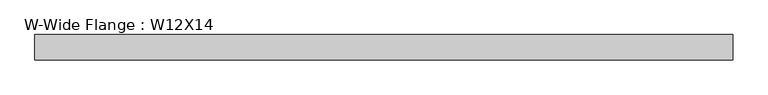
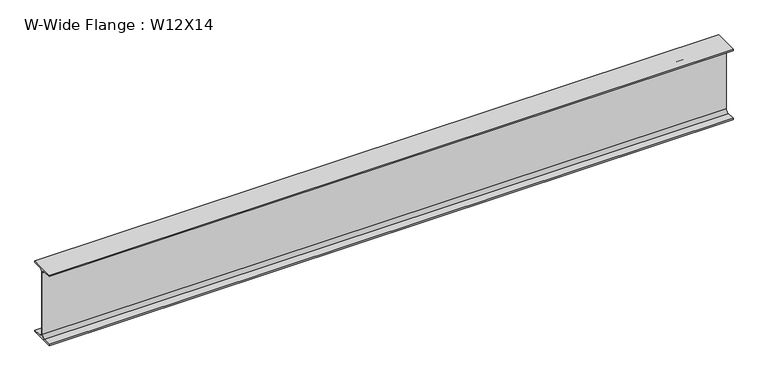
"""IFC4 building model written with IfcOpenShell, lengths in millimetres: beam geometry, W-Wide Flange : W12X14."""

from ifc_helpers import new_model, si_unit, point, frame, frame_2d, origin, place, context, project, spatial, polyline, circle_curve, trimmed, segment, composite_curve, outline, extrude, source, transform, mapped, element, save


def w_wide_flange_w12x14_1f2f6d33(model_context):
    return source(origin(), model_context, "Body", "SweptSolid", [
        extrude(outline(composite_curve([segment(polyline([(50.419, -145.415), (50.419, -151.13), (-50.419, -151.13), (-50.419, -145.415), (-15.875, -145.415)]), True, "CONTINUOUS"), segment(trimmed(circle_curve(frame_2d((-15.875, -132.08)), 13.335), [point((-15.875, -145.415))], [point((-2.54, -132.08))], True, "CARTESIAN"), True, "CONTINUOUS"), segment(polyline([(-2.54, -132.08), (-2.54, 132.08)]), True, "CONTINUOUS"), segment(trimmed(circle_curve(frame_2d((-15.875, 132.08)), 13.335), [point((-2.54, 132.08))], [point((-15.875, 145.415))], True, "CARTESIAN"), True, "CONTINUOUS"), segment(polyline([(-15.875, 145.415), (-50.419, 145.415), (-50.419, 151.13), (50.419, 151.13), (50.419, 145.415), (15.875, 145.415)]), True, "CONTINUOUS"), segment(trimmed(circle_curve(frame_2d((15.875, 132.08)), 13.335), [point((15.875, 145.415))], [point((2.54, 132.08))], True, "CARTESIAN"), True, "CONTINUOUS"), segment(polyline([(2.54, 132.08), (2.54, -132.08)]), True, "CONTINUOUS"), segment(trimmed(circle_curve(frame_2d((15.875, -132.08)), 13.335), [point((2.54, -132.08))], [point((15.875, -145.415))], True, "CARTESIAN"), True, "CONTINUOUS"), segment(polyline([(15.875, -145.415), (50.419, -145.415)]), True, "CONTINUOUS")], self_intersect=False)), frame((-1370.33, 0.0, 0.0), z_axis=(1.0, 0.0, 0.0), x_axis=(0.0, 1.0, 0.0)), (0.0, 0.0, 1.0), 2770.759),
    ])


if __name__ == "__main__":
    model = new_model("IFC4")
    model_context = context("Model", 3, world=origin())
    ifc_project = project(units=[si_unit("LENGTHUNIT", "METRE", prefix="MILLI")], contexts=[model_context])
    site = spatial("IfcSite", under=ifc_project)
    building = spatial("IfcBuilding", under=site)
    placement = place(None, origin())
    w_wide_flange_w12x14_shape = w_wide_flange_w12x14_1f2f6d33(model_context)
    element("IfcBeam", 1, ObjectType="W-Wide Flange : W12X14", at=placement, inside=building, context=model_context, shape_type="MappedRepresentation", body=[
        mapped(w_wide_flange_w12x14_shape, transform((0.0, 0.0, 0.0), x_axis=(1.0, 0.0, 0.0), y_axis=(0.0, 1.0, 0.0), z_axis=(0.0, 0.0, 1.0))),
    ])
    save(model, "model.ifc")

# Revit data of these elements
# Type "W-Wide Flange : W12X14"
#   Assembly Code = "B10"
#   W = 14
#   Length [instance default] = 5' - 0"
#   bf = 0' - 3.97"
#   d = 0' - 11.9"
#   k = 0' - 0 3/4"
#   k2 = 0' - 0.525"
#   tf = 0' - 0.225"
#   tw = 0' - 0.2"
#   A = 0.0288889 SF
#   Structural Material [instance default] = Steel ASTM A992
# Element 1 (IfcBeam, "W-Wide Flange : W12X14")
#   Materials on its faces: "Steel ASTM A992"
# Materials
#   "Steel ASTM A992": class "Metal", colour RGB 199 199 199, transparency 0, Description = "Structural steel 50ksi", Cost = 0
